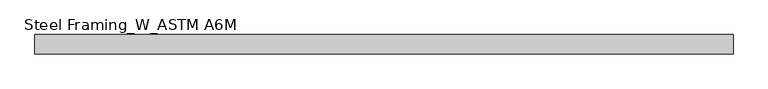
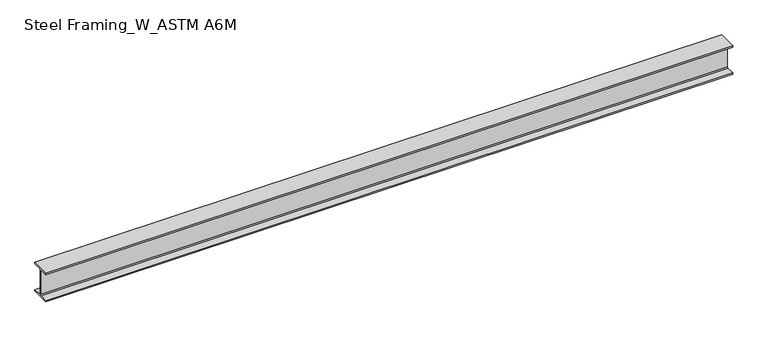
"""IFC4 building model written with IfcOpenShell, lengths in millimetres: beam geometry, Steel Framing_W_ASTM A6M : H_SB_AR_S02_W200x31.3_RB4."""

from ifc_helpers import new_model, si_unit, point, frame, frame_2d, origin, place, context, project, spatial, polyline, circle_curve, trimmed, segment, composite_curve, outline, extrude, source, transform, mapped, element, save


def steel_framing_w_astm_a6m_19955ad1(model_context):
    return source(origin(), model_context, "Body", "SweptSolid", [
        extrude(outline(composite_curve([segment(polyline([(67.0, -94.8), (67.0, -105.0), (-67.0, -105.0), (-67.0, -94.8), (-10.775, -94.8)]), True, "CONTINUOUS"), segment(trimmed(circle_curve(frame_2d((-10.775, -87.2)), 7.6), [point((-10.775, -94.8))], [point((-3.175, -87.2))], True, "CARTESIAN"), True, "CONTINUOUS"), segment(polyline([(-3.175, -87.2), (-3.175, 87.2)]), True, "CONTINUOUS"), segment(trimmed(circle_curve(frame_2d((-10.775, 87.2)), 7.6), [point((-3.175, 87.2))], [point((-10.775, 94.8))], True, "CARTESIAN"), True, "CONTINUOUS"), segment(polyline([(-10.775, 94.8), (-67.0, 94.8), (-67.0, 105.0), (67.0, 105.0), (67.0, 94.8), (10.775, 94.8)]), True, "CONTINUOUS"), segment(trimmed(circle_curve(frame_2d((10.775, 87.2)), 7.6), [point((10.775, 94.8))], [point((3.175, 87.2))], True, "CARTESIAN"), True, "CONTINUOUS"), segment(polyline([(3.175, 87.2), (3.175, -87.2)]), True, "CONTINUOUS"), segment(trimmed(circle_curve(frame_2d((10.775, -87.2)), 7.6), [point((3.175, -87.2))], [point((10.775, -94.8))], True, "CARTESIAN"), True, "CONTINUOUS"), segment(polyline([(10.775, -94.8), (67.0, -94.8)]), True, "CONTINUOUS")], self_intersect=False)), frame((-2399.9, 0.0, 0.0), z_axis=(1.0, 0.0, 0.0), x_axis=(0.0, 1.0, 0.0)), (0.0, 0.0, 1.0), 4799.8),
    ])


if __name__ == "__main__":
    model = new_model("IFC4")
    model_context = context("Model", 3, world=origin())
    ifc_project = project(units=[si_unit("LENGTHUNIT", "METRE", prefix="MILLI")], contexts=[model_context])
    site = spatial("IfcSite", under=ifc_project)
    building = spatial("IfcBuilding", under=site)
    placement = place(None, origin())
    steel_framing_w_astm_a6m_shape = steel_framing_w_astm_a6m_19955ad1(model_context)
    element("IfcBeam", 1, ObjectType="Steel Framing_W_ASTM A6M : H_SB_AR_S02_W200x31.3_RB4", at=placement, inside=building, context=model_context, shape_type="MappedRepresentation", body=[
        mapped(steel_framing_w_astm_a6m_shape, transform((0.0, 0.0, 0.0), x_axis=(1.0, 0.0, 0.0), y_axis=(0.0, 1.0, 0.0), z_axis=(0.0, 0.0, 1.0))),
    ])
    save(model, "model.ifc")

# Revit data of these elements
# Type "Steel Framing_W_ASTM A6M : H_SB_AR_S02_W200x31.3_RB4"
#   Type Mark = "RB4"
#   Section Name Key = "W8x21"
#   Width = 13.4 cm
#   Web Thickness = 0.635 cm
#   Web Fillet = 0.76 cm
#   Warping Constant = 40800.0 cm⁶
#   Torsional Moment of Inertia = 11.70 cm⁴
#   Section Area = 39.7 cm²
#   Plastic Modulus weak axis = 93.2 cm³
#   Plastic Modulus strong axis = 334.0 cm³
#   Perimeter = 0.93 m²/m
#   Nominal Weight = 31.30 kgf/m
#   Moment of Inertia weak axis = 407.00 cm⁴
#   Moment of Inertia strong axis = 3130.00 cm⁴
#   Height = 21.0 cm
#   Flange Thickness = 1.02 cm
#   Elastic Modulus weak axis = 60.8 cm³
#   Elastic Modulus strong axis = 298.0 cm³
#   Centroid Vertical = 10.5 cm
#   Centroid Horizontal = 6.7 cm
#   Length [instance default] = 1500 mm
#   Structural Material [instance default] = Steel, 45-345
#   Bolt Spacing = 0
#   Assembly Code = ""
# Element 1 (IfcBeam, "Steel Framing_W_ASTM A6M : H_SB_AR_S02_W200x31.3_RB4")
#   Materials on its faces: "Steel, 45-345"
# Materials
#   "Steel, 45-345": class "Metal", colour RGB 189 187 185, transparency 0, Description = "Steel 345 MPa", Cost = 0
